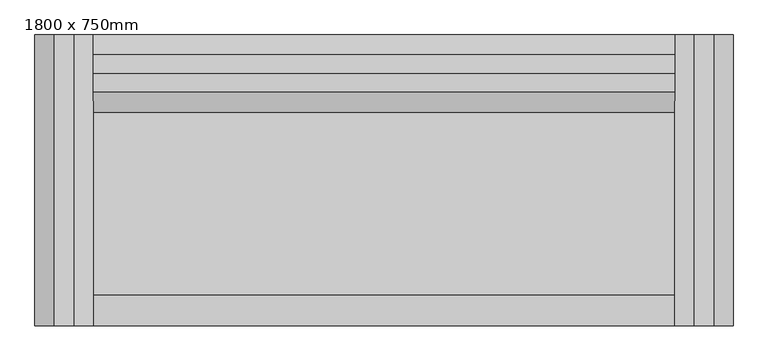
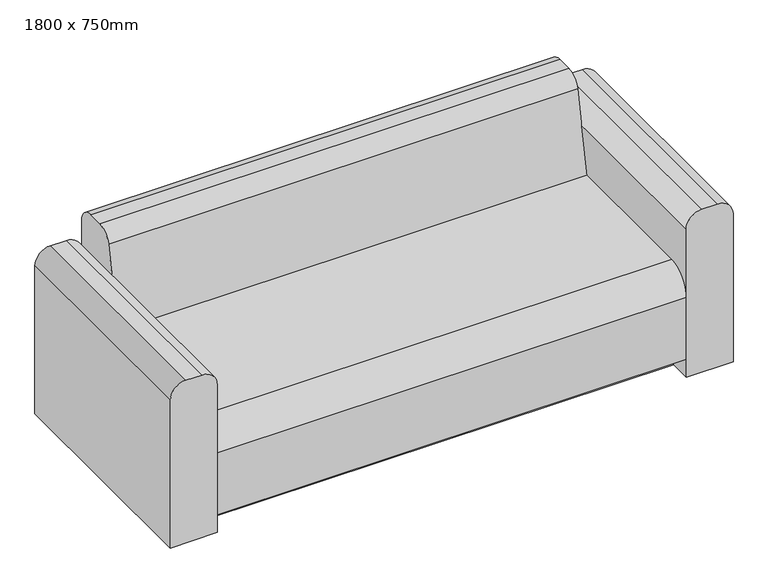
"""IFC4 building model written with IfcOpenShell, lengths in millimetres: furniture geometry, ソファ－I型 : 1800 x 750mm."""

from ifc_helpers import new_model, si_unit, point, frame, frame_2d, origin, place, context, project, spatial, polyline, circle_curve, trimmed, segment, composite_curve, outline, extrude, source, transform, mapped, element, save


def furniture_1800_x_750mm_b4778df9(model_context):
    return source(origin(), model_context, "Body", "SweptSolid", [
        extrude(outline(composite_curve([segment(trimmed(circle_curve(frame_2d((500.0, -850.0)), 50.0), [point((550.0, -850.0))], [point((500.0, -900.0))], False, "CARTESIAN"), True, "CONTINUOUS"), segment(polyline([(500.0, -900.0), (0.0, -900.0), (0.0, -750.0), (500.0, -750.0)]), True, "CONTINUOUS"), segment(trimmed(circle_curve(frame_2d((500.0, -800.0)), 50.0), [point((500.0, -750.0))], [point((550.0, -800.0))], False, "CARTESIAN"), True, "CONTINUOUS"), segment(polyline([(550.0, -800.0), (550.0, -850.0)]), True, "CONTINUOUS")], self_intersect=False)), frame((0.0, -375.0, 0.0), z_axis=(0.0, 1.0, 0.0), x_axis=(0.0, 0.0, 1.0)), (0.0, 0.0, 1.0), 750.0),
        extrude(outline(composite_curve([segment(polyline([(550.0, 850.0), (550.0, 800.0)]), True, "CONTINUOUS"), segment(trimmed(circle_curve(frame_2d((500.0, 800.0)), 50.0), [point((550.0, 800.0))], [point((500.0, 750.0))], False, "CARTESIAN"), True, "CONTINUOUS"), segment(polyline([(500.0, 750.0), (0.0, 750.0), (0.0, 900.0), (500.0, 900.0)]), True, "CONTINUOUS"), segment(trimmed(circle_curve(frame_2d((500.0, 850.0)), 50.0), [point((500.0, 900.0))], [point((550.0, 850.0))], False, "CARTESIAN"), True, "CONTINUOUS")], self_intersect=False)), frame((0.0, -375.0, 0.0), z_axis=(0.0, 1.0, 0.0), x_axis=(0.0, 0.0, 1.0)), (0.0, 0.0, 1.0), 750.0),
        extrude(outline(composite_curve([segment(trimmed(circle_curve(frame_2d((275.9901951, 600.0)), 50.0), [point((226.9611614, 609.8058068))], [point((275.9901951, 650.0))], False, "CARTESIAN"), True, "CONTINUOUS"), segment(polyline([(275.9901951, 650.0), (325.0, 650.0)]), True, "CONTINUOUS"), segment(trimmed(circle_curve(frame_2d((325.0, 600.0)), 50.0), [point((325.0, 650.0))], [point((375.0, 600.0))], False, "CARTESIAN"), True, "CONTINUOUS"), segment(polyline([(375.0, 600.0), (375.0, 0.0), (-305.0, 0.0), (-305.0, 60.0), (-375.0, 60.0), (-375.0, 270.0)]), True, "CONTINUOUS"), segment(trimmed(circle_curve(frame_2d((-295.0, 270.0)), 80.0), [point((-375.0, 270.0))], [point((-295.0, 350.0))], False, "CARTESIAN"), True, "CONTINUOUS"), segment(polyline([(-295.0, 350.0), (175.0, 350.0), (226.9611614, 609.8058068)]), True, "CONTINUOUS")], self_intersect=False)), frame((-750.0, 0.0, 0.0), z_axis=(1.0, 0.0, 0.0), x_axis=(0.0, 1.0, 0.0)), (0.0, 0.0, 1.0), 1500.0),
    ])


if __name__ == "__main__":
    model = new_model("IFC4")
    model_context = context("Model", 3, world=origin())
    ifc_project = project(units=[si_unit("LENGTHUNIT", "METRE", prefix="MILLI")], contexts=[model_context])
    site = spatial("IfcSite", under=ifc_project)
    building = spatial("IfcBuilding", under=site)
    placement = place(None, origin())
    furniture_1800_x_750mm_shape = furniture_1800_x_750mm_b4778df9(model_context)
    element("IfcFurniture", 1, ObjectType="ソファ－I型 : 1800 x 750mm", at=placement, inside=building, context=model_context, shape_type="MappedRepresentation", body=[
        mapped(furniture_1800_x_750mm_shape, transform((0.0, 0.0, 0.0), x_axis=(1.0, 0.0, 0.0), y_axis=(0.0, 1.0, 0.0), z_axis=(0.0, 0.0, 1.0))),
    ])
    save(model, "model.ifc")

# Revit data of these elements
# Type "ソファ－I型 : 1800 x 750mm"
#   Keynote = "12490.Y1"
#   座面高さ = 350 mm
#   幅 = 1800 mm
#   奥行き = 750 mm
#   本体 = モチアミ - 無地 - グレー
#   Default Elevation = 0
# Element 1 (IfcFurniture, "ソファ－I型 : 1800 x 750mm")
#   Materials on its faces: "モチアミ - 無地 - グレー"
# Materials
#   "モチアミ - 無地 - グレー": class "モチアミ", colour RGB 65 63 65, transparency 0, Cost = 0
